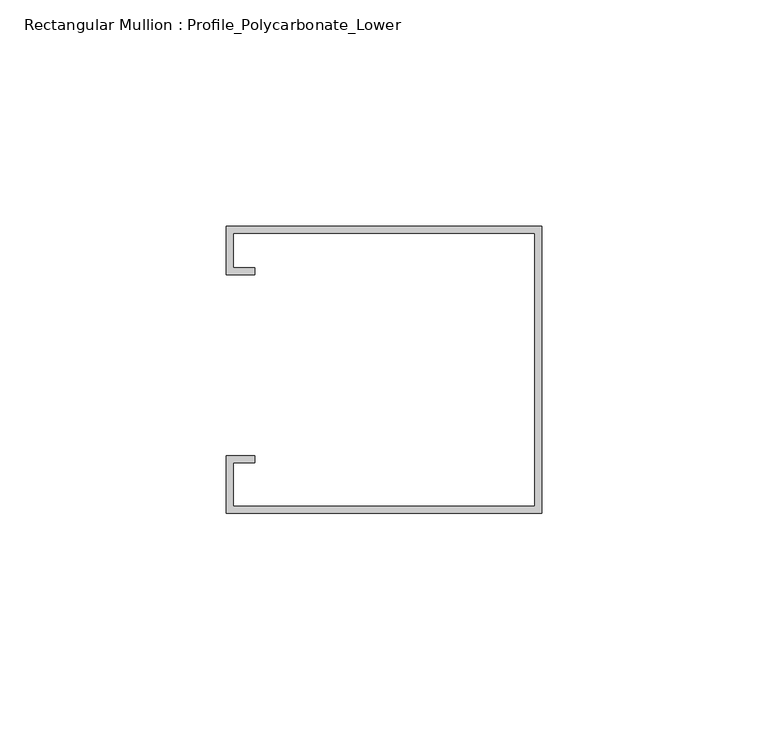
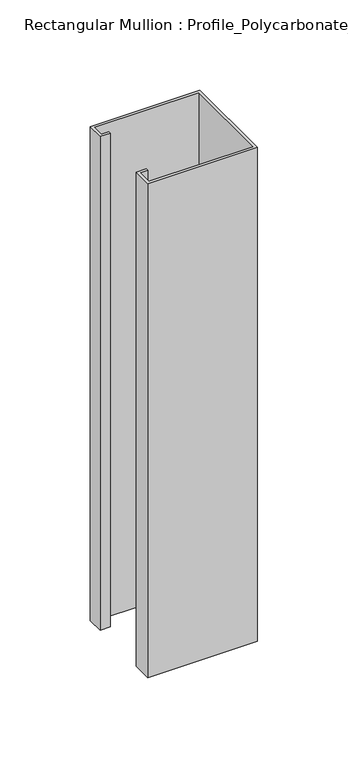
"""IFC4 building model written with IfcOpenShell, lengths in millimetres: member geometry, Rectangular Mullion : Profile_Polycarbonate_Lower."""

from ifc_helpers import new_model, si_unit, frame, origin, place, context, project, spatial, polyline, outline, extrude, source, transform, mapped, element, save


def rectangular_mullion_profile_polycarbonate_lower_e83f1224(model_context):
    return source(origin(), model_context, "Body", "SweptSolid", [
        extrude(outline(polyline([(0.0, -32.7), (-69.85, -32.7), (-69.85, -20.0), (-63.5, -20.0), (-63.5, -21.5875), (-68.2625, -21.5875), (-68.2625, -31.1125), (-1.5875, -31.1125), (-1.5875, 29.2125), (-68.2625, 29.2125), (-68.2625, 21.5875), (-63.5, 21.5875), (-63.5, 20.0), (-69.85, 20.0), (-69.85, 30.8), (0.0, 30.8), (0.0, -32.7)])), frame((0.0, 0.0, -333.375), z_axis=(0.0, 0.0, 1.0), x_axis=(1.0, 0.0, 0.0)), (0.0, 0.0, 1.0), 333.375),
    ])


if __name__ == "__main__":
    model = new_model("IFC4")
    model_context = context("Model", 3, world=origin())
    ifc_project = project(units=[si_unit("LENGTHUNIT", "METRE", prefix="MILLI")], contexts=[model_context])
    site = spatial("IfcSite", under=ifc_project)
    building = spatial("IfcBuilding", under=site)
    placement = place(None, origin())
    rectangular_mullion_profile_polycarbonate_lower_shape = rectangular_mullion_profile_polycarbonate_lower_e83f1224(model_context)
    element("IfcMember", 1, ObjectType="Rectangular Mullion : Profile_Polycarbonate_Lower", at=placement, inside=building, context=model_context, shape_type="MappedRepresentation", body=[
        mapped(rectangular_mullion_profile_polycarbonate_lower_shape, transform((0.0, 0.0, 0.0), x_axis=(1.0, 0.0, 0.0), y_axis=(0.0, 1.0, 0.0), z_axis=(0.0, 0.0, 1.0))),
    ])
    save(model, "model.ifc")

# Revit data of these elements
# Type "Rectangular Mullion : Profile_Polycarbonate_Lower"
#   built-in parameter 1007322 = 0.208333 (stored number, unit not read)
#   built-in parameter 1007321 = 0 (stored number, unit not read)
#   built-in parameter 1007320 = 0.00520833 (stored number, unit not read)
# Element 1 (IfcMember, "Rectangular Mullion : Profile_Polycarbonate_Lower")
#   Materials on its faces: "GALVANIZED UNISTRUT P5500, 1 5/8\" X 2 7/16\" OR ALUM. CHANNEL"
# Materials
#   "GALVANIZED UNISTRUT P5500, 1 5/8\" X 2 7/16\" OR ALUM. CHANNEL": class "Metal", colour RGB 244 244 244, transparency 0, Description = "Aluminum 6061", Cost = 0
